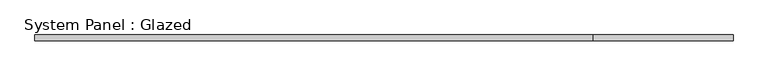
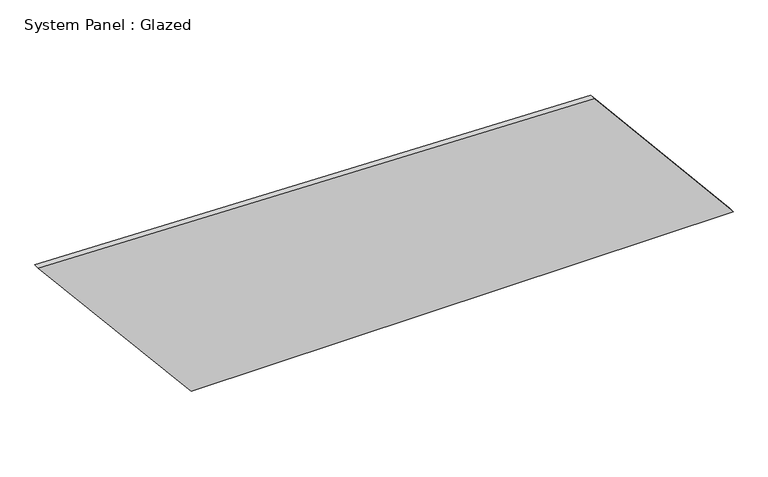
"""IFC4 building model written with IfcOpenShell, lengths in millimetres: plate geometry, System Panel : Glazed."""

from ifc_helpers import new_model, si_unit, frame, origin, place, context, project, spatial, polyline, outline, extrude, source, transform, mapped, element, save


def system_panel_glazed_95e458a9(model_context):
    return source(origin(), model_context, "Body", "SweptSolid", [
        extrude(outline(polyline([(0.0, -810.878799), (0.0, 1447.4931417), (700.2647225, 868.0544709), (764.2779696, -1447.4931417), (0.0, -810.878799)])), frame((0.0, -49.5, 0.0), z_axis=(0.0, 1.0, 0.0), x_axis=(0.0, 0.0, 1.0)), (0.0, 0.0, 1.0), 25.0),
    ])


if __name__ == "__main__":
    model = new_model("IFC4")
    model_context = context("Model", 3, world=origin())
    ifc_project = project(units=[si_unit("LENGTHUNIT", "METRE", prefix="MILLI")], contexts=[model_context])
    site = spatial("IfcSite", under=ifc_project)
    building = spatial("IfcBuilding", under=site)
    placement = place(None, origin())
    system_panel_glazed_shape = system_panel_glazed_95e458a9(model_context)
    element("IfcPlate", 1, ObjectType="System Panel : Glazed", at=placement, inside=building, context=model_context, shape_type="MappedRepresentation", body=[
        mapped(system_panel_glazed_shape, transform((0.0, 0.0, 0.0), x_axis=(1.0, 0.0, 0.0), y_axis=(0.0, 1.0, 0.0), z_axis=(0.0, 0.0, 1.0))),
    ])
    save(model, "model.ifc")

# Revit data of these elements
# Element 1 (IfcPlate, "System Panel : Glazed")
#   Materials on its faces: "Glass, Clear Glazing"
# Materials
#   "Glass, Clear Glazing": class "Glass", colour RGB 247 249 248, transparency 0.85, Description = "Clear glazing", Cost = 0
